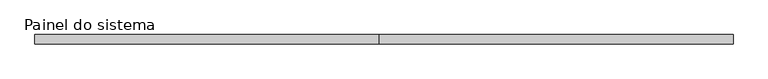
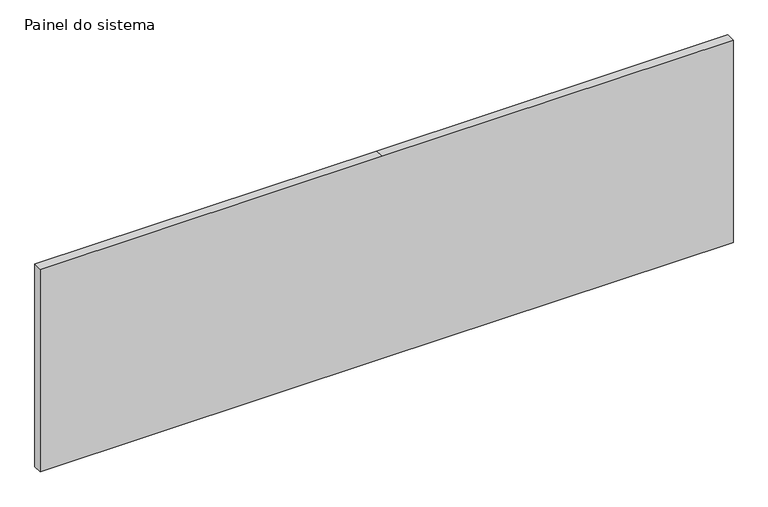
"""IFC4 building model written with IfcOpenShell, lengths in millimetres: plate geometry, Painel do sistema : Envidraçado."""

from ifc_helpers import new_model, si_unit, frame, origin, place, context, project, spatial, polyline, outline, extrude, source, transform, mapped, element, save


def painel_do_sistema_b3a4ee0d(model_context):
    return source(origin(), model_context, "Body", "SweptSolid", [
        extrude(outline(polyline([(0.0, -954.2100001), (0.0, -12.4999998), (0.0, 954.2100001), (590.0, 954.2100001), (590.0, -12.4999998), (590.0, -954.2100001), (0.0, -954.2100001)])), frame((0.0, -49.5, 0.0), z_axis=(0.0, 1.0, 0.0), x_axis=(0.0, 0.0, 1.0)), (0.0, 0.0, 1.0), 25.0),
    ])


if __name__ == "__main__":
    model = new_model("IFC4")
    model_context = context("Model", 3, world=origin())
    ifc_project = project(units=[si_unit("LENGTHUNIT", "METRE", prefix="MILLI")], contexts=[model_context])
    site = spatial("IfcSite", under=ifc_project)
    building = spatial("IfcBuilding", under=site)
    placement = place(None, origin())
    painel_do_sistema_shape = painel_do_sistema_b3a4ee0d(model_context)
    element("IfcPlate", 1, ObjectType="Painel do sistema : Envidraçado", at=placement, inside=building, context=model_context, shape_type="MappedRepresentation", body=[
        mapped(painel_do_sistema_shape, transform((0.0, 0.0, 0.0), x_axis=(1.0, 0.0, 0.0), y_axis=(0.0, 1.0, 0.0), z_axis=(0.0, 0.0, 1.0))),
    ])
    save(model, "model.ifc")

# Revit data of these elements
# Type "Painel do sistema : Envidraçado"
#   Construction Type Id = "GSP4R"
#   Analytic Construction = "Vidraça única Pilkington 1/8 pol"
#   Visual Light Transmittance = 0.9
#   Solar Heat Gain Coefficient = 0.86
#   Heat Transfer Coefficient (U) = 6.7069 W/(m²·K)
# Element 1 (IfcPlate, "Painel do sistema : Envidraçado")
#   Materials on its faces: ".VIDRO GENÉRICO"
# Materials
#   ".VIDRO GENÉRICO": class ".CC_VIDRO", colour RGB 0 128 192, transparency 0.9, Description = "Vidro comum", Cost = 0
